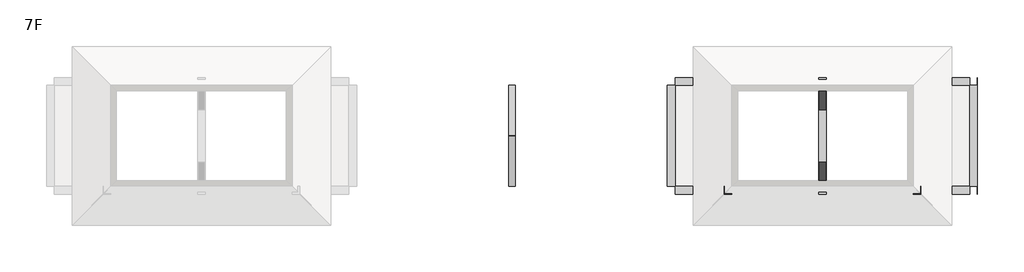
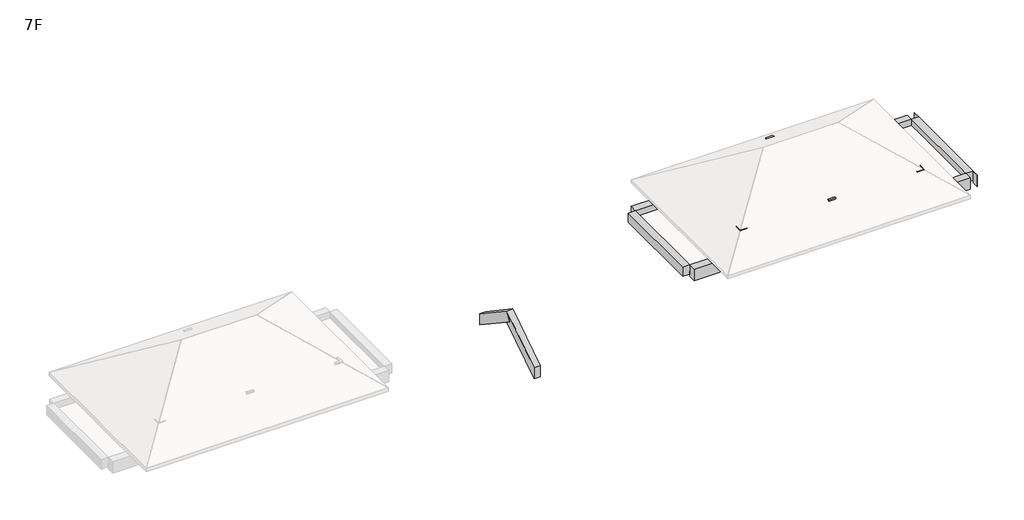
# One storey, part 2 of 2: 17 beams, 7 columns, 1 proxy.
"""IFC4 building model written with IfcOpenShell, lengths in millimetres."""

import ifcopenshell
import ifcopenshell.guid

model = None  # the IFC model being written
_history = None  # IfcOwnerHistory: only IFC2X3 demands one
_inside = {}  # id of a spatial element -> (the spatial element, [elements in it])
_under = {}  # id of a project, library or spatial element -> (it, [spatial elements below it])
_declared = {}  # id of a project -> (the project, [libraries it declares])
_typed = {}  # id of a type object -> (the type object, [elements of that type])
_made_of = {}  # id of a material, layer set ... -> (it, [elements and type objects made of it])


def new_model(schema):
    """Start an empty IFC model of exactly this schema.

    Asked for "IFC4X3", IfcOpenShell would pick the latest addendum, in which some entities
    have other attributes; the version numbers below select the first issue.
    IFC2X3 requires an IfcOwnerHistory on every rooted entity: one is made here for all.
    """
    global model, _history
    if schema == "IFC4X3":
        model = ifcopenshell.file(schema_version=(4, 3, 0, 0))
    else:
        model = ifcopenshell.file(schema=schema)
    _inside.clear()
    _under.clear()
    _declared.clear()
    _typed.clear()
    _made_of.clear()
    _history = None
    if model.schema == "IFC2X3":
        org = make("IfcOrganization", Name="unknown")
        user = make(
            "IfcPersonAndOrganization",
            ThePerson=make("IfcPerson", FamilyName="unknown"),
            TheOrganization=org,
        )
        app = make(
            "IfcApplication",
            ApplicationDeveloper=org,
            Version="unknown",
            ApplicationFullName="unknown",
            ApplicationIdentifier="unknown",
        )
        _history = make(
            "IfcOwnerHistory",
            OwningUser=user,
            OwningApplication=app,
            ChangeAction="ADDED",
            CreationDate=0,
        )
    return model


def make(cls, **values):
    """One entity of the class cls with the attributes given. An attribute that is None is left unset."""
    return model.create_entity(
        cls, **{name: value for name, value in values.items() if value is not None}
    )


def rooted(cls, **values):
    """An entity with a GlobalId (a new one), such as an element, a storey or a relation."""
    return make(cls, GlobalId=ifcopenshell.guid.new(), OwnerHistory=_history, **values)


def si_unit(unit_type, name, prefix=None):
    """IfcSIUnit, for example si_unit("LENGTHUNIT", "METRE", prefix="MILLI")."""
    return make("IfcSIUnit", UnitType=unit_type, Prefix=prefix, Name=name)


def assignment(units):
    """IfcUnitAssignment: the units of a project."""
    return None if units is None else make("IfcUnitAssignment", Units=units)


def point(xyz):
    """IfcCartesianPoint."""
    return None if xyz is None else make("IfcCartesianPoint", Coordinates=xyz)


def direction(xyz):
    """IfcDirection."""
    return None if xyz is None else make("IfcDirection", DirectionRatios=xyz)


def frame(location, z_axis=None, x_axis=None):
    """IfcAxis2Placement3D, a coordinate frame: its origin and axes. An axis left out is left unset."""
    return make(
        "IfcAxis2Placement3D",
        Location=point(location),
        Axis=direction(z_axis),
        RefDirection=direction(x_axis),
    )


def frame_2d(location, x_axis=None):
    """IfcAxis2Placement2D, a coordinate frame in the plane: its origin and x axis."""
    return make(
        "IfcAxis2Placement2D", Location=point(location), RefDirection=direction(x_axis)
    )


def origin():
    """The frame at (0, 0, 0) with its axes left unset."""
    return frame((0.0, 0.0, 0.0))


def origin_with_axes():
    """The frame at (0, 0, 0) with the z axis (0, 0, 1) and the x axis (1, 0, 0) written out."""
    return frame((0.0, 0.0, 0.0), z_axis=(0.0, 0.0, 1.0), x_axis=(1.0, 0.0, 0.0))


def place(relative_to, where):
    """IfcLocalPlacement: puts the frame where relative to a parent placement (None: the world)."""
    return make(
        "IfcLocalPlacement", PlacementRelTo=relative_to, RelativePlacement=where
    )


def context(
    kind, dimensions, precision=None, world=None, true_north=None, identifier=None
):
    """IfcGeometricRepresentationContext, for example the 3D "Model" context."""
    return make(
        "IfcGeometricRepresentationContext",
        ContextIdentifier=identifier,
        ContextType=kind,
        CoordinateSpaceDimension=dimensions,
        Precision=precision,
        WorldCoordinateSystem=world,
        TrueNorth=true_north,
    )


def project(units=None, contexts=None):
    """IfcProject with its units and contexts."""
    return rooted(
        "IfcProject",
        Name="project",
        RepresentationContexts=contexts,
        UnitsInContext=assignment(units),
    )


def spatial(cls, under=None, at=None, **own):
    """A site, building, storey or space (cls), placed at a placement, below another one or the project."""
    s = rooted(cls, ObjectPlacement=at, **own)
    if under is not None:
        _under.setdefault(under.id(), (under, []))[1].append(s)
    return s


def polyline(points):
    """IfcPolyline through the points."""
    return make("IfcPolyline", Points=[point(p) for p in points])


def circle_curve(where, radius):
    """IfcCircle in the frame where."""
    return make("IfcCircle", Position=where, Radius=radius)


def ellipse_curve(where, semi_axis1, semi_axis2):
    """IfcEllipse in the frame where."""
    return make(
        "IfcEllipse", Position=where, SemiAxis1=semi_axis1, SemiAxis2=semi_axis2
    )


def trimmed(basis, trim1, trim2, sense, master):
    """IfcTrimmedCurve: the piece of a basis curve between two trims."""
    return make(
        "IfcTrimmedCurve",
        BasisCurve=basis,
        Trim1=trim1,
        Trim2=trim2,
        SenseAgreement=sense,
        MasterRepresentation=master,
    )


def segment(curve, same_sense, transition):
    """IfcCompositeCurveSegment."""
    return make(
        "IfcCompositeCurveSegment",
        Transition=transition,
        SameSense=same_sense,
        ParentCurve=curve,
    )


def composite_curve(segments, self_intersect=None):
    """IfcCompositeCurve: segments joined end to end."""
    return make("IfcCompositeCurve", Segments=segments, SelfIntersect=self_intersect)


def outline(outer, holes=None, kind="AREA"):
    """IfcArbitraryClosedProfileDef: a profile drawn as a closed curve; with holes, ...WithVoids."""
    if holes is None:
        return make("IfcArbitraryClosedProfileDef", ProfileType=kind, OuterCurve=outer)
    return make(
        "IfcArbitraryProfileDefWithVoids",
        ProfileType=kind,
        OuterCurve=outer,
        InnerCurves=holes,
    )


def extrude(swept, where, along, depth):
    """IfcExtrudedAreaSolid: the profile swept, set in the frame where, extruded along a direction by depth."""
    return make(
        "IfcExtrudedAreaSolid",
        SweptArea=swept,
        Position=where,
        ExtrudedDirection=direction(along),
        Depth=depth,
    )


def faces_of(points, faces, orient=None, outer=None):
    """IfcFace entities. A face is a list of loops; a loop is a list of indices into points, from 0.

    orient and outer hold one flag for each loop. By default every Orientation is true, the
    first loop of a face is its IfcFaceOuterBound and the others are IfcFaceBound.
    """
    made = []
    for i, loops in enumerate(faces):
        bounds = []
        for j, loop in enumerate(loops):
            is_outer = j == 0 if outer is None else outer[i][j]
            bounds.append(
                make(
                    "IfcFaceOuterBound" if is_outer else "IfcFaceBound",
                    Bound=make("IfcPolyLoop", Polygon=[points[k] for k in loop]),
                    Orientation=True if orient is None else orient[i][j],
                )
            )
        made.append(make("IfcFace", Bounds=bounds))
    return made


def faceted_brep(points, faces, orient=None, outer=None, voids=None):
    """IfcFacetedBrep: a solid bounded by flat faces; with voids (closed shells), ...WithVoids."""
    shared = [point(p) for p in points]
    hull = make("IfcClosedShell", CfsFaces=faces_of(shared, faces, orient, outer))
    if voids is None:
        return make("IfcFacetedBrep", Outer=hull)
    return make(
        "IfcFacetedBrepWithVoids",
        Outer=hull,
        Voids=[
            make(cls, CfsFaces=faces_of(shared, fs, o, b)) for cls, fs, o, b in voids
        ],
    )


def shape(context_of_items, identifier, shape_type, items):
    """IfcShapeRepresentation: the items that make up one representation, for example the "Body"."""
    return make(
        "IfcShapeRepresentation",
        ContextOfItems=context_of_items,
        RepresentationIdentifier=identifier,
        RepresentationType=shape_type,
        Items=items,
    )


def source(mapping_origin, context_of_items, identifier, shape_type, items):
    """IfcRepresentationMap: a shape defined once, which mapped items show again and again."""
    return make(
        "IfcRepresentationMap",
        MappingOrigin=mapping_origin,
        MappedRepresentation=shape(context_of_items, identifier, shape_type, items),
    )


def transform(
    local_origin,
    x_axis=None,
    y_axis=None,
    z_axis=None,
    scale=None,
    scale2=None,
    scale3=None,
    uniform=True,
):
    """IfcCartesianTransformationOperator3D, or its non-uniform kind. x_axis, y_axis, z_axis: its Axis1, 2, 3."""
    if uniform:
        return make(
            "IfcCartesianTransformationOperator3D",
            Axis1=direction(x_axis),
            Axis2=direction(y_axis),
            LocalOrigin=point(local_origin),
            Scale=scale,
            Axis3=direction(z_axis),
        )
    return make(
        "IfcCartesianTransformationOperator3DnonUniform",
        Axis1=direction(x_axis),
        Axis2=direction(y_axis),
        LocalOrigin=point(local_origin),
        Scale=scale,
        Axis3=direction(z_axis),
        Scale2=scale2,
        Scale3=scale3,
    )


def mapped(mapping_source, mapping_target):
    """IfcMappedItem: shows the shape of a source again, moved by a transform."""
    return make(
        "IfcMappedItem", MappingSource=mapping_source, MappingTarget=mapping_target
    )


def made_of(thing, what):
    """Note that an element or type object is made of a material, layer set ...; save() writes the relation."""
    if what is not None:
        _made_of.setdefault(what.id(), (what, []))[1].append(thing)
    return thing


def element(
    cls,
    number,
    at=None,
    inside=None,
    cuts=None,
    type_object=None,
    material=None,
    context=None,
    identifier="Body",
    shape_type=None,
    held_by="IfcProductDefinitionShape",
    body=None,
    shapes=None,
    **own,
):
    """One element of the class cls, such as IfcWall. Its Tag is "e" and its number.

    at: its placement. inside: the storey or other place that contains it. cuts: it is an
    opening in that element (IfcRelVoidsElement). A single representation is given by context,
    identifier, shape_type and body (its items); several are given by shapes. held_by: the class
    of the entity that holds the representations. save() writes the other relations.
    """
    e = rooted(cls, Tag="e%d" % number, ObjectPlacement=at, **own)
    if body is not None:
        shapes = [shape(context, identifier, shape_type, body)]
    if shapes is not None:
        e.Representation = make(held_by, Representations=shapes)
    if inside is not None:
        _inside.setdefault(inside.id(), (inside, []))[1].append(e)
    if cuts is not None:
        rooted(
            "IfcRelVoidsElement", RelatingBuildingElement=cuts, RelatedOpeningElement=e
        )
    if type_object is not None:
        _typed.setdefault(type_object.id(), (type_object, []))[1].append(e)
    return made_of(e, material)


def aggregate(whole, parts):
    """IfcRelAggregates: a whole, such as a stair, and the parts it consists of."""
    return rooted("IfcRelAggregates", RelatingObject=whole, RelatedObjects=parts)


def save(model, path):
    """Write the relations noted so far, then the file.

    IfcRelAggregates (storeys below a building ...), IfcRelContainedInSpatialStructure (elements
    in a storey), IfcRelDefinesByType, IfcRelAssociatesMaterial and IfcRelDeclares: one each for
    every whole, place, type object, material and project.
    """
    for whole, parts in _under.values():
        aggregate(whole, parts)
    for where, things in _inside.values():
        rooted(
            "IfcRelContainedInSpatialStructure",
            RelatedElements=things,
            RelatingStructure=where,
        )
    for kind, things in _typed.values():
        rooted("IfcRelDefinesByType", RelatedObjects=things, RelatingType=kind)
    for what, things in _made_of.values():
        rooted("IfcRelAssociatesMaterial", RelatedObjects=things, RelatingMaterial=what)
    for by, libraries in _declared.values():
        rooted("IfcRelDeclares", RelatingContext=by, RelatedDefinitions=libraries)
    model.write(path)


def plane_surface(at):
    """IfcPlane: the flat surface through the origin of the frame at, square to its z axis."""
    return make("IfcPlane", Position=at)


def cylinder_surface(at, radius):
    """IfcCylindricalSurface: all points at the distance radius from the z axis of the frame at."""
    return make("IfcCylindricalSurface", Position=at, Radius=radius)


def revolved_surface(curve, axis_point, axis_direction):
    """IfcSurfaceOfRevolution: the curve turned about the line through axis_point along axis_direction."""
    return make(
        "IfcSurfaceOfRevolution",
        SweptCurve=make("IfcArbitraryOpenProfileDef", ProfileType="CURVE", Curve=curve),
        AxisPosition=make("IfcAxis1Placement", Location=point(axis_point), Axis=direction(axis_direction)),
    )


def advanced_brep(points, edges, surfaces, faces):
    """IfcAdvancedBrep: a solid bounded by faces that lie on surfaces and meet in shared edges.

    An edge is (start, end): straight between two places in points (the first is 0);
    or (start, end, curve); or (start, end, curve, False) where it runs against its curve.
    A face is (place in surfaces, loops), or (place, loops, False) where it looks against
    its surface's normal. A loop lists edges by number (the first is 1), with a minus sign
    where the edge is run from its end to its start. The first loop is the outer one.
    """
    corners = [point(p) for p in points]
    vertices = [make("IfcVertexPoint", VertexGeometry=c) for c in corners]
    made = []
    for start, end, *more in edges:
        made.append(
            make(
                "IfcEdgeCurve",
                EdgeStart=vertices[start],
                EdgeEnd=vertices[end],
                EdgeGeometry=more[0] if more else make("IfcPolyline", Points=[corners[start], corners[end]]),
                SameSense=more[1] if len(more) > 1 else True,
            )
        )
    hull = []
    for where, loops, *sense in faces:
        bounds = []
        for j, loop in enumerate(loops):
            ring = [make("IfcOrientedEdge", EdgeElement=made[abs(k) - 1], Orientation=k > 0) for k in loop]
            bounds.append(
                make(
                    "IfcFaceOuterBound" if j == 0 else "IfcFaceBound",
                    Bound=make("IfcEdgeLoop", EdgeList=ring),
                    Orientation=True,
                )
            )
        hull.append(make("IfcAdvancedFace", Bounds=bounds, FaceSurface=surfaces[where], SameSense=sense[0] if sense else True))
    return make("IfcAdvancedBrep", Outer=make("IfcClosedShell", CfsFaces=hull))


def m_support_metal_circular_m_support_metal_circular_a779fbb7(model_context):
    return source(origin(), model_context, "Body", "SolidModel", [
        advanced_brep(
        [(-6.0, 0.0, 0.0), (6.0, 0.0, 0.0), (-6.0, 0.0, -63.0), (6.0, 0.0, -63.0), (6.0, 12.0, -75.0), (-6.0, 12.0, -75.0), (-6.0, 63.0, -75.0), (6.0, 63.0, -75.0)],
        [
            (0, 1, circle_curve(origin_with_axes(), 6.0)),
            (1, 0, circle_curve(origin_with_axes(), 6.0)),
            (0, 2),
            (2, 3, circle_curve(frame((0.0, 0.0, -63.0), z_axis=(0.0, 0.0, 1.0), x_axis=(1.0, 0.0, 0.0)), 6.0)),
            (3, 1),
            (3, 2, circle_curve(frame((0.0, 0.0, -63.0), z_axis=(0.0, 0.0, 1.0), x_axis=(1.0, 0.0, 0.0)), 6.0)),
            (4, 3, circle_curve(frame((6.0, 12.0, -63.0), z_axis=(-1.0, 0.0, 0.0), x_axis=(0.0, -1.0, 0.0)), 12.0)),
            (2, 5, circle_curve(frame((-6.0, 12.0, -63.0), z_axis=(1.0, 0.0, 0.0), x_axis=(0.0, -1.0, 0.0)), 12.0)),
            (5, 4, circle_curve(frame((0.0, 12.0, -75.0), z_axis=(0.0, -1.0, 0.0), x_axis=(1.0, 0.0, 0.0)), 6.0)),
            (4, 5, circle_curve(frame((0.0, 12.0, -75.0), z_axis=(0.0, -1.0, 0.0), x_axis=(1.0, 0.0, 0.0)), 6.0)),
            (6, 7, circle_curve(frame((0.0, 63.0, -75.0), z_axis=(0.0, 1.0, 0.0), x_axis=(1.0, 0.0, 0.0)), 6.0)),
            (7, 6, circle_curve(frame((0.0, 63.0, -75.0), z_axis=(0.0, 1.0, 0.0), x_axis=(1.0, 0.0, 0.0)), 6.0)),
            (5, 6),
            (7, 4),
        ],
        [
            plane_surface(origin_with_axes()),
            cylinder_surface(origin_with_axes(), 6.0),
            revolved_surface(trimmed(ellipse_curve(frame((0.0, 0.0, -63.0), z_axis=(0.0, 0.0, 1.0), x_axis=(1.0, 0.0, 0.0)), 6.0, 6.0), [point((-6.0, 0.0, -63.0))], [point((6.0, 0.0, -63.0))], True, "CARTESIAN"), (0.0, 12.0, -63.0), (1.0, 0.0, 0.0)),
            revolved_surface(trimmed(ellipse_curve(frame((0.0, 0.0, -63.0), z_axis=(0.0, 0.0, 1.0), x_axis=(1.0, 0.0, 0.0)), 6.0, 6.0), [point((6.0, 0.0, -63.0))], [point((-6.0, 0.0, -63.0))], True, "CARTESIAN"), (0.0, 12.0, -63.0), (1.0, 0.0, 0.0)),
            plane_surface(frame((0.0, 63.0, -75.0), z_axis=(0.0, 1.0, 0.0), x_axis=(1.0, 0.0, 0.0))),
            cylinder_surface(frame((0.0, 12.0, -75.0), z_axis=(0.0, -1.0, 0.0), x_axis=(1.0, 0.0, 0.0)), 6.0),
        ],
        [
            (0, [[1, 2]]),
            (1, [[-1, 3, 4, 5]]),
            (1, [[-2, -5, 6, -3]]),
            (2, [[7, -4, 8, 9]]),
            (3, [[-8, -6, -7, 10]]),
            (4, [[11, 12]]),
            (5, [[-9, 13, -12, 14]]),
            (5, [[-10, -14, -11, -13]]),
        ],
    ),
        extrude(outline(composite_curve([segment(trimmed(circle_curve(frame_2d((-75.0, 0.0)), 25.0), [point((-75.0, -25.0))], [point((-75.0, 25.0))], False, "CARTESIAN"), True, "CONTINUOUS"), segment(trimmed(circle_curve(frame_2d((-75.0, 0.0)), 25.0), [point((-75.0, 25.0))], [point((-75.0, -25.0))], False, "CARTESIAN"), True, "CONTINUOUS")], self_intersect=False)), frame((0.0, 63.0, 0.0), z_axis=(0.0, 1.0, 0.0), x_axis=(0.0, 0.0, 1.0)), (0.0, 0.0, 1.0), 12.0),
    ])


model = new_model("IFC4")

# Units and contexts
model_context = context("Model", 3, world=origin())
ifc_project = project(units=[si_unit("LENGTHUNIT", "METRE", prefix="MILLI")], contexts=[model_context])

# Site, building, storey
site = spatial("IfcSite", under=ifc_project)
building = spatial("IfcBuilding", under=site)
storey = spatial("IfcBuildingStorey", under=building, Name="7F", Elevation=20530.0)

# Beams
placement = place(None, origin())
element("IfcBeam", 1, ObjectType="M_Concrete-Rectangular Beam : 250x400", at=placement, inside=storey, context=model_context, shape_type="Brep", body=[
    faceted_brep([(17975.0000046, 8450.0000002, 18285.6270793), (17725.0000046, 8450.0000002, 18285.6270793), (17725.0000046, 6499.7375861, 19585.8347272), (17975.0000046, 6499.7375861, 19585.8347272), (17725.0000046, 8450.0000002, 17804.8831884), (17725.0000046, 6499.7375861, 19105.0908362), (17725.0000046, 6277.8536437, 19253.0171854), (17975.0000046, 8450.0000002, 17804.8831884), (17975.0000046, 6499.7375861, 19105.0908362), (17975.0000046, 6277.8536437, 19253.0171854)], [[[0, 1, 2, 3]], [[4, 5, 6, 2, 1]], [[6, 5, 4, 7, 8, 9]], [[3, 9, 8, 7, 0]], [[1, 0, 7, 4]], [[3, 2, 6, 9]]]),
])
element("IfcBeam", 2, ObjectType="M_Concrete-Rectangular Beam : 250x400", at=placement, inside=storey, context=model_context, shape_type="SweptSolid", body=[
    extrude(outline(polyline([(33399.8746483, 8449.9999997), (33649.8746483, 8449.9999997), (33649.8746483, 4549.9999996), (33399.8746483, 4549.9999996), (33399.8746483, 8449.9999997)])), frame((0.0, 0.0, 20130.0), z_axis=(0.0, 0.0, 1.0), x_axis=(1.0, 0.0, 0.0)), (0.0, 0.0, 1.0), 400.0),
])
element("IfcBeam", 3, ObjectType="M_Concrete-Rectangular Beam : 250x400", at=placement, inside=storey, context=model_context, shape_type="SweptSolid", body=[
    extrude(outline(polyline([(26050.1253733, 8449.9999997), (26300.1253733, 8449.9999997), (26300.1253733, 4549.9999996), (26050.1253733, 4549.9999996), (26050.1253733, 8449.9999997)])), frame((0.0, 0.0, 20130.0), z_axis=(0.0, 0.0, 1.0), x_axis=(1.0, 0.0, 0.0)), (0.0, 0.0, 1.0), 400.0),
])
element("IfcBeam", 4, ObjectType="M_Concrete-Rectangular Beam : 250x400", at=placement, inside=storey, context=model_context, shape_type="SweptSolid", body=[
    extrude(outline(polyline([(4550.0000005, 18285.9769737), (6499.7375861, 19585.8347272), (6277.8536437, 19253.0171854), (6499.7375861, 19105.0908362), (4550.0000005, 17805.2330827), (4550.0000005, 18285.9769737)])), frame((17725.0000046, 0.0, 0.0), z_axis=(1.0, 0.0, 0.0), x_axis=(0.0, 1.0, 0.0)), (0.0, 0.0, 1.0), 250.0),
])
element("IfcBeam", 5, ObjectType="M_Concrete-Rectangular Beam : 250x400", at=placement, inside=storey, context=model_context, shape_type="Brep", body=[
    faceted_brep([(29725.0000715, 6499.7375861, 22885.8347272), (29975.0000715, 6499.7375861, 22885.8347272), (29975.0000715, 8449.9999997, 21585.6270796), (29725.0000715, 8449.9999997, 21585.6270796), (29725.0000715, 6277.8536437, 22553.0171854), (29725.0000715, 8449.9999997, 21104.8831887), (29725.0000715, 6499.7375861, 22405.0908362), (29975.0000715, 6277.8536437, 22553.0171854), (29975.0000715, 8449.9999997, 21104.8831887), (29975.0000715, 6499.7375861, 22405.0908362)], [[[0, 1, 2, 3]], [[4, 0, 3, 5, 6]], [[7, 4, 6, 5, 8, 9]], [[1, 7, 9, 8, 2]], [[1, 0, 4, 7]], [[3, 2, 8, 5]]]),
])
element("IfcBeam", 6, ObjectType="M_Concrete-Rectangular Beam : 250x400", at=placement, inside=storey, context=model_context, shape_type="SweptSolid", body=[
    extrude(outline(polyline([(6277.8536437, 22553.0171854), (6499.7375861, 22405.0908362), (4549.9999992, 21105.2330819), (4549.9999992, 21585.9769728), (6499.7375861, 22885.8347272), (6277.8536437, 22553.0171854)])), frame((29725.0000715, 0.0, 0.0), z_axis=(1.0, 0.0, 0.0), x_axis=(0.0, 1.0, 0.0)), (0.0, 0.0, 1.0), 250.0),
])
element("IfcBeam", 7, ObjectType="M_Concrete-Rectangular Beam : 250x400", at=placement, inside=storey, context=model_context, shape_type="Brep", body=[
    faceted_brep([(33629.982566, 4549.9999992, 21480.0), (33629.982566, 8724.9999993, 21480.0), (33625.119648, 8724.9999993, 21480.0), (33508.5592163, 8608.4366337, 21480.0), (33379.982566, 8608.4366337, 21480.0), (33379.982566, 8474.9999993, 21480.0), (33379.982566, 4549.9999992, 21480.0), (33379.982566, 4549.9999992, 21080.0), (33379.982566, 8655.7227157, 21448.4751524), (33379.982566, 8474.9999993, 21448.4751524), (33379.982566, 8449.9999997, 21448.4751524), (33379.982566, 8449.9999997, 21080.0), (33629.982566, 4549.9999992, 21080.0), (33629.982566, 8449.9999997, 21080.0), (33629.982566, 8449.9999997, 21448.4751524), (33629.982566, 8724.9999993, 21448.4751524), (33625.119648, 8724.9999993, 21448.4751524), (33555.8441081, 8655.7227157, 21448.4751524)], [[[0, 1, 2, 3, 4, 5, 6]], [[7, 6, 5, 4, 8, 9, 10, 11]], [[12, 7, 11, 13]], [[1, 0, 12, 13, 14, 15]], [[1, 15, 16, 2]], [[0, 6, 7, 12]], [[10, 14, 13, 11]], [[14, 10, 9, 8, 17, 16, 15]], [[3, 17, 8, 4]], [[17, 3, 2, 16]]]),
])
element("IfcBeam", 8, ObjectType="M_Concrete-Rectangular Beam : 250x400", at=placement, inside=storey, context=model_context, shape_type="SweptSolid", body=[
    extrude(outline(polyline([(21080.0, 26075.0175606), (21080.0, 26325.0175606), (21480.0, 26325.0175606), (21480.0, 26191.5713244), (21402.3014348, 26075.0175606), (21080.0, 26075.0175606)])), frame((0.0, 4549.9999992, 0.0), z_axis=(0.0, 1.0, 0.0), x_axis=(0.0, 0.0, 1.0)), (0.0, 0.0, 1.0), 3887.3000005),
])
element("IfcBeam", 9, ObjectType="M_Concrete-Rectangular Beam : 250x400", at=placement, inside=storey, context=model_context, shape_type="Brep", body=[
    faceted_brep([(29999.9855437, 8474.9999993, 21480.0), (33379.982566, 8474.9999993, 21480.0), (33379.982566, 8608.4366337, 21480.0), (29999.9855437, 8608.4366337, 21480.0), (33379.982566, 8474.9999993, 21448.4751524), (29999.9855437, 8474.9999993, 21080.0), (33349.8746414, 8474.9999993, 21080.0), (33349.8746414, 8474.9999993, 21448.4751524), (33349.8746414, 8724.9999993, 21080.0), (29999.9855437, 8724.9999993, 21080.0), (29999.9855437, 8724.9999993, 21402.2891349), (33349.8746414, 8724.9999993, 21402.2891349), (33379.982566, 8655.7227157, 21448.4751524), (33349.8746414, 8655.7227157, 21448.4751524)], [[[0, 1, 2, 3]], [[4, 1, 0, 5, 6, 7]], [[8, 6, 5, 9]], [[8, 9, 10, 11]], [[1, 4, 12, 2]], [[7, 6, 8, 11, 13]], [[4, 7, 13, 12]], [[5, 0, 3, 10, 9]], [[3, 2, 12, 13, 11, 10]]]),
    faceted_brep([(26075.0175606, 8474.9999993, 21448.4751524), (26075.0175606, 8474.9999993, 21480.0), (26075.0175606, 8724.7509238, 21480.0), (26075.0175606, 8724.7509238, 21448.4751524), (26350.1253663, 8474.9999993, 21080.0), (26350.1253663, 8474.9999993, 21448.4751524), (26350.1253663, 8655.7227157, 21448.4751524), (26350.1253663, 8724.9999993, 21402.2891349), (26350.1253663, 8724.9999993, 21080.0), (26144.0475062, 8655.7227157, 21448.4751524), (29699.9855437, 8474.9999993, 21480.0), (29699.9855437, 8474.9999993, 21080.0), (29699.9855437, 8724.9999993, 21080.0), (29699.9855437, 8724.9999993, 21402.2891349), (29699.9855437, 8608.4366337, 21480.0), (26191.3347784, 8608.4366337, 21480.0)], [[[0, 1, 2, 3]], [[4, 5, 6, 7, 8]], [[5, 0, 3, 9, 6]], [[10, 11, 12, 13, 14]], [[1, 10, 14, 15, 2]], [[1, 0, 5, 4, 11, 10]], [[4, 8, 12, 11]], [[12, 8, 7, 13]], [[15, 9, 3, 2]], [[9, 15, 14, 13, 7, 6]]]),
])
element("IfcBeam", 10, ObjectType="M_Concrete-Rectangular Beam : 250x400", at=placement, inside=storey, context=model_context, shape_type="SweptSolid", body=[
    extrude(outline(polyline([(4524.9999902, 21080.0), (4274.9999902, 21080.0), (4274.9999902, 21402.6390255), (4391.0385331, 21480.0), (4524.9999902, 21480.0), (4524.9999902, 21080.0)])), frame((29999.9855437, 0.0, 0.0), z_axis=(1.0, 0.0, 0.0), x_axis=(0.0, 1.0, 0.0)), (0.0, 0.0, 1.0), 3349.8890977),
    extrude(outline(polyline([(4524.9999902, 21480.0), (4524.9999902, 21080.0), (4274.9999902, 21080.0), (4274.9999902, 21402.6390255), (4391.0385331, 21480.0), (4524.9999902, 21480.0)])), frame((26350.0175606, 0.0, 0.0), z_axis=(1.0, 0.0, 0.0), x_axis=(0.0, 1.0, 0.0)), (0.0, 0.0, 1.0), 3349.9679831),
])
element("IfcBeam", 11, ObjectType="M_Concrete-Rectangular Beam : 300x400", at=placement, inside=storey, context=model_context, shape_type="Brep", body=[
    faceted_brep([(30000.0000031, 8449.9999997, 20530.0), (29999.533537, 8449.9999997, 20530.0), (29700.0000031, 8449.9999997, 20530.0), (29700.0000031, 4549.9999996, 20530.0), (29999.533537, 4549.9999996, 20530.0), (30000.0000031, 4549.9999996, 20530.0), (29700.0000031, 8449.9999997, 20130.0), (29700.0000031, 4549.9999996, 20130.0), (30000.0000031, 8449.9999997, 20130.0), (30000.0000031, 4549.9999996, 20130.0)], [[[0, 1, 2, 3, 4, 5]], [[2, 6, 7, 3]], [[6, 8, 9, 7]], [[8, 0, 5, 9]], [[2, 1, 0, 8, 6]], [[5, 4, 3, 7, 9]]]),
])
element("IfcBeam", 12, ObjectType="M_Concrete-Rectangular Beam : 300x400", at=placement, inside=storey, context=model_context, shape_type="Brep", body=[
    faceted_brep([(35835.035019, 8449.9999997, 20530.0), (35834.4843149, 8449.9999997, 20530.0), (35535.035019, 8449.9999997, 20530.0), (35535.035019, 4549.9999996, 20530.0), (35834.4843149, 4549.9999996, 20530.0), (35835.035019, 4549.9999996, 20530.0), (35535.035019, 8449.9999997, 20130.0), (35535.035019, 4549.9999996, 20130.0), (35835.035019, 8449.9999997, 20130.0), (35835.035019, 4549.9999996, 20130.0)], [[[0, 1, 2, 3, 4, 5]], [[2, 6, 7, 3]], [[6, 8, 9, 7]], [[8, 0, 5, 9]], [[2, 1, 0, 8, 6]], [[5, 4, 3, 7, 9]]]),
])
element("IfcBeam", 13, ObjectType="M_Concrete-Rectangular Beam : 300x400", at=placement, inside=storey, context=model_context, shape_type="Brep", body=[
    faceted_brep([(24149.9825174, 8449.9999997, 20530.0), (24149.516027, 8449.9999997, 20530.0), (23849.9825174, 8449.9999997, 20530.0), (23849.9825174, 4550.0000005, 20530.0), (24149.516027, 4549.9999996, 20530.0), (24149.9825174, 4549.9999996, 20530.0), (23849.9825174, 8449.9999997, 20130.0), (23849.9825174, 4550.0000005, 20130.0), (24149.9825174, 8449.9999997, 20130.0), (24149.9825174, 4549.9999996, 20130.0)], [[[0, 1, 2, 3, 4, 5]], [[2, 6, 7, 3]], [[6, 8, 9, 7]], [[8, 0, 5, 9]], [[2, 1, 0, 8, 6]], [[3, 7, 9, 5, 4]]]),
])
element("IfcBeam", 14, ObjectType="M_Concrete-Rectangular Beam : 300x500", at=placement, inside=storey, context=model_context, shape_type="Brep", body=[
    faceted_brep([(30000.0000031, 8449.9999997, 20530.0), (30000.0000031, 8749.9999997, 20530.0), (29999.533537, 8749.9999997, 20530.0), (29999.533537, 8449.9999997, 20530.0), (30000.0000031, 8449.9999997, 20030.0), (30000.0000031, 8449.9999997, 20130.0), (29999.533537, 8449.9999997, 20030.0), (30000.0000031, 8749.9999997, 20030.0), (29999.533537, 8749.9999997, 20030.0)], [[[0, 1, 2, 3]], [[4, 5, 0, 3, 6]], [[7, 4, 6, 8]], [[1, 7, 8, 2]], [[1, 0, 5, 4, 7]], [[3, 2, 8, 6]]]),
    faceted_brep([(24149.516027, 8449.9999997, 20530.0), (24149.516027, 8749.9999997, 20530.0), (24149.516027, 8749.9999997, 20030.0), (24149.516027, 8449.9999997, 20030.0), (29699.533537, 8749.9999997, 20530.0), (29699.533537, 8449.9999997, 20530.0), (29699.533537, 8449.9999997, 20030.0), (29699.533537, 8749.9999997, 20030.0), (24149.9825174, 8449.9999997, 20530.0), (26050.1253733, 8449.9999997, 20530.0), (26300.1253733, 8449.9999997, 20530.0), (26350.1253663, 8449.9999997, 20530.0), (26350.1253663, 8749.9999997, 20530.0), (26050.1253663, 8749.9999997, 20530.0)], [[[0, 1, 2, 3]], [[4, 5, 6, 7]], [[1, 0, 8, 9, 10, 11, 5, 4, 12, 13]], [[0, 3, 6, 5, 11, 10, 9, 8]], [[3, 2, 7, 6]], [[2, 1, 13, 12, 4, 7]]]),
])
element("IfcBeam", 15, ObjectType="M_Concrete-Rectangular Beam : 300x500", at=placement, inside=storey, context=model_context, shape_type="Brep", body=[
    faceted_brep([(30000.0000031, 4249.9999996, 20530.0), (30000.0000031, 4549.9999996, 20530.0), (29999.533537, 4549.9999996, 20530.0), (29999.533537, 4249.9999996, 20530.0), (30000.0000031, 4249.9999996, 20030.0), (29999.533537, 4249.9999996, 20030.0), (30000.0000031, 4549.9999996, 20030.0), (29999.533537, 4549.9999996, 20030.0), (30000.0000031, 4549.9999996, 20130.0)], [[[0, 1, 2, 3]], [[4, 0, 3, 5]], [[6, 4, 5, 7]], [[1, 8, 6, 7, 2]], [[1, 0, 4, 6, 8]], [[3, 2, 7, 5]]]),
    faceted_brep([(24149.516027, 4249.9999996, 20530.0), (24149.516027, 4549.9999996, 20530.0), (24149.516027, 4549.9999996, 20030.0), (24149.516027, 4249.9999996, 20030.0), (29699.533537, 4549.9999996, 20530.0), (29699.533537, 4249.9999996, 20530.0), (29699.533537, 4249.9999996, 20030.0), (29699.533537, 4549.9999996, 20030.0), (26300.1253733, 4549.9999996, 20530.0), (26050.1253733, 4549.9999996, 20530.0), (24149.9825174, 4549.9999996, 20530.0)], [[[0, 1, 2, 3]], [[4, 5, 6, 7]], [[1, 0, 5, 4, 8, 9, 10]], [[0, 3, 6, 5]], [[3, 2, 7, 6]], [[2, 1, 10, 9, 8, 4, 7]]]),
])
element("IfcBeam", 16, ObjectType="M_Concrete-Rectangular Beam : 300x500", at=placement, inside=storey, context=model_context, shape_type="Brep", body=[
    faceted_brep([(35835.035019, 8449.9999997, 20530.0), (35835.035019, 8749.9999997, 20530.0), (35834.4843149, 8749.9999997, 20530.0), (35834.4843149, 8449.9999997, 20530.0), (35835.035019, 8449.9999997, 20030.0), (35835.035019, 8449.9999997, 20130.0), (35834.4843149, 8449.9999997, 20030.0), (35835.035019, 8749.9999997, 20030.0), (35834.4843149, 8749.9999997, 20030.0)], [[[0, 1, 2, 3]], [[4, 5, 0, 3, 6]], [[7, 4, 6, 8]], [[1, 7, 8, 2]], [[1, 0, 5, 4, 7]], [[3, 2, 8, 6]]]),
    faceted_brep([(35534.4843149, 8749.9999997, 20530.0), (35534.4843149, 8449.9999997, 20530.0), (35534.4843149, 8449.9999997, 20030.0), (35534.4843149, 8749.9999997, 20030.0), (30000.0000031, 8449.9999997, 20530.0), (30000.0000031, 8749.9999997, 20530.0), (30000.0000031, 8749.9999997, 20030.0), (30000.0000031, 8449.9999997, 20030.0), (33349.8746414, 8449.9999997, 20530.0), (33399.8746483, 8449.9999997, 20530.0), (33649.8746483, 8449.9999997, 20530.0), (33649.8746414, 8749.9999997, 20530.0), (33349.8746414, 8749.9999997, 20530.0)], [[[0, 1, 2, 3]], [[4, 5, 6, 7]], [[5, 4, 8, 9, 10, 1, 0, 11, 12]], [[4, 7, 2, 1, 10, 9, 8]], [[7, 6, 3, 2]], [[6, 5, 12, 11, 0, 3]]]),
])
element("IfcBeam", 17, ObjectType="M_Concrete-Rectangular Beam : 300x500", at=placement, inside=storey, context=model_context, shape_type="Brep", body=[
    faceted_brep([(35835.035019, 4249.9999996, 20530.0), (35835.035019, 4549.9999996, 20530.0), (35834.4843149, 4549.9999996, 20530.0), (35834.4843149, 4249.9999996, 20530.0), (35835.035019, 4249.9999996, 20030.0), (35834.4843149, 4249.9999996, 20030.0), (35835.035019, 4549.9999996, 20030.0), (35834.4843149, 4549.9999996, 20030.0), (35835.035019, 4549.9999996, 20130.0)], [[[0, 1, 2, 3]], [[4, 0, 3, 5]], [[6, 4, 5, 7]], [[1, 8, 6, 7, 2]], [[1, 0, 4, 6, 8]], [[3, 2, 7, 5]]]),
    faceted_brep([(30000.0000031, 4249.9999996, 20530.0), (30000.0000031, 4549.9999996, 20530.0), (30000.0000031, 4549.9999996, 20030.0), (30000.0000031, 4249.9999996, 20030.0), (35534.4843149, 4549.9999996, 20530.0), (35534.4843149, 4249.9999996, 20530.0), (35534.4843149, 4249.9999996, 20030.0), (35534.4843149, 4549.9999996, 20030.0), (33649.8746483, 4549.9999996, 20530.0), (33399.8746483, 4549.9999996, 20530.0)], [[[0, 1, 2, 3]], [[4, 5, 6, 7]], [[5, 4, 8, 9, 1, 0]], [[6, 5, 0, 3]], [[7, 6, 3, 2]], [[4, 7, 2, 1, 9, 8]]]),
])

# Proxy
m_support_metal_circular_m_support_metal_circular_shape = m_support_metal_circular_m_support_metal_circular_a779fbb7(model_context)
element("IfcBuildingElementProxy", 18, Name="M_Support - Metal - Circular : M_Support - Metal - Circular", ObjectType="M_Support - Metal - Circular : M_Support - Metal - Circular", at=placement, inside=storey, context=model_context, shape_type="MappedRepresentation", body=[
    mapped(m_support_metal_circular_m_support_metal_circular_shape, transform((4604.999959, 3949.9999996, 20530.0), x_axis=(1.0, 0.0, 0.0), y_axis=(0.0, 1.0, 0.0), z_axis=(0.0, 0.0, 1.0))),
])

# Columns
element("IfcColumn", 19, ObjectType="M_Concrete-Rectangular-Column : 300x300", at=placement, inside=storey, context=model_context, shape_type="SweptSolid", body=[
    extrude(outline(polyline([(9649.8746382, 8749.9999997), (9649.8746382, 8449.9999997), (9349.8746382, 8449.9999997), (9349.8746382, 8749.9999997), (9649.8746382, 8749.9999997)])), frame((0.0, 0.0, 20530.0), z_axis=(0.0, 0.0, 1.0), x_axis=(1.0, 0.0, 0.0)), (0.0, 0.0, 1.0), 918.4751524),
])
element("IfcColumn", 20, ObjectType="M_Concrete-Rectangular-Column : 300x300", at=placement, inside=storey, context=model_context, shape_type="Brep", body=[
    faceted_brep([(29999.9855437, 4549.9999992, 20530.0), (29999.9855437, 4249.9999992, 20530.0), (29699.9855437, 4249.9999992, 20530.0), (29699.9855437, 4549.9999992, 20530.0), (29699.9855437, 4549.9999992, 21585.9769764), (29999.9855437, 4549.9999992, 21585.9769764), (29999.9855437, 4249.9999992, 21385.9719455), (29999.9855437, 4274.9999902, 21402.6390255), (29999.9855437, 4391.0385331, 21480.0), (29699.9855437, 4391.0385331, 21480.0), (29699.9855437, 4274.9999902, 21402.6390255), (29699.9855437, 4249.9999992, 21385.9719455)], [[[0, 1, 2, 3]], [[0, 3, 4, 5]], [[6, 7, 8, 5, 4, 9, 10, 11]], [[1, 0, 5, 8, 7, 6]], [[2, 1, 6, 11]], [[3, 2, 11, 10, 9, 4]]]),
    faceted_brep([(29999.9855437, 4249.9999992, 21585.9769764), (29999.9855437, 4249.9999992, 21530.1951128), (29999.9855437, 4333.6706899, 21585.9769764), (29699.9855437, 4249.9999992, 21585.9769764), (29699.9855437, 4249.9999992, 21530.1951128), (29699.9855437, 4333.6706899, 21585.9769764)], [[[0, 1, 2]], [[0, 3, 4, 1]], [[4, 3, 5]], [[3, 0, 2, 5]], [[2, 1, 4, 5]]]),
])
element("IfcColumn", 21, ObjectType="M_Concrete-Rectangular-Column : 300x300", at=placement, inside=storey, context=model_context, shape_type="Brep", body=[
    faceted_brep([(29999.9855437, 8749.9999997, 20530.0), (29999.9855437, 8449.9999997, 20530.0), (29999.533537, 8449.9999997, 20530.0), (29699.9855437, 8449.9999997, 20530.0), (29699.9855437, 8749.9999997, 20530.0), (29999.533537, 8749.9999997, 20530.0), (29999.9855437, 8449.9999997, 21585.6270796), (29699.9855437, 8449.9999997, 21585.6270796), (29999.9855437, 8608.4366337, 21480.0), (29999.9855437, 8724.9999993, 21402.2891349), (29999.9855437, 8749.9999997, 21385.6220487), (29699.9855437, 8749.9999997, 21385.6220487), (29699.9855437, 8724.9999993, 21402.2891349), (29699.9855437, 8608.4366337, 21480.0)], [[[0, 1, 2, 3, 4, 5]], [[3, 2, 1, 6, 7]], [[6, 8, 9, 10, 11, 12, 13, 7]], [[1, 0, 10, 9, 8, 6]], [[4, 3, 7, 13, 12, 11]], [[0, 5, 4, 11, 10]]]),
    faceted_brep([(29999.9855437, 8749.9999997, 21529.845216), (29999.9855437, 8749.9999997, 21585.6270796), (29999.9855437, 8666.329309, 21585.6270796), (29699.9855437, 8749.9999997, 21585.6270796), (29699.9855437, 8749.9999997, 21529.845216), (29699.9855437, 8666.329309, 21585.6270796)], [[[0, 1, 2]], [[3, 4, 5]], [[3, 1, 0, 4]], [[1, 3, 5, 2]], [[0, 2, 5, 4]]]),
])
element("IfcColumn", 22, ObjectType="M_Concrete-Rectangular-Column : 300x300", at=placement, inside=storey, context=model_context, shape_type="Brep", body=[
    faceted_brep([(33649.8746414, 4549.9999992, 20530.0), (33649.8746414, 4249.9999992, 20530.0), (33349.8746414, 4249.9999992, 20530.0), (33349.8746414, 4549.9999992, 20530.0), (33649.8746414, 4549.9999992, 21544.0553738), (33649.8746414, 4249.9999992, 21544.0553738), (33649.8746414, 4249.9999992, 21529.9272796), (33649.8746414, 4549.9999992, 21529.9272796), (33649.8746414, 4249.9999992, 21385.7074809), (33649.5942023, 4249.9999992, 21385.8944308), (33649.5942023, 4249.9999992, 21530.1142294), (33349.8746414, 4249.9999992, 21544.0553738), (33349.8746414, 4549.9999992, 21544.0553738), (33628.6814244, 4549.9999992, 21544.0553738), (33628.6814244, 4270.9133035, 21544.0553738), (33412.3407455, 4487.2594281, 21544.0553738), (33412.3407455, 4549.9999992, 21544.0553738), (33649.8746414, 4549.9999992, 21385.7074809)], [[[0, 1, 2, 3]], [[4, 5, 6, 7]], [[2, 1, 8, 9, 10, 6, 5, 11]], [[3, 2, 11, 12]], [[4, 7, 13]], [[5, 4, 13, 14, 15, 16, 12, 11]], [[15, 9, 8, 17, 16]], [[10, 14, 13, 7, 6]], [[9, 15, 14, 10]], [[1, 0, 17, 8]], [[0, 3, 12, 16, 17]]]),
])
element("IfcColumn", 23, ObjectType="M_Concrete-Rectangular-Column : 300x300", at=placement, inside=storey, context=model_context, shape_type="Brep", body=[
    faceted_brep([(33649.8746414, 8749.9999997, 20530.0), (33649.8746414, 8449.9999997, 20530.0), (33349.8746414, 8449.9999997, 20530.0), (33349.8746414, 8749.9999997, 20530.0), (33649.8746414, 8749.9999997, 21385.6220487), (33649.8746414, 8749.7556157, 21385.7849755), (33649.8746414, 8749.7556157, 21448.4751524), (33649.8746414, 8449.9999997, 21448.4751524), (33349.8746414, 8449.9999997, 21448.4751524), (33349.8746414, 8655.7227157, 21448.4751524), (33349.8746414, 8749.9999997, 21385.6220487), (33555.8441081, 8655.7227157, 21448.4751524)], [[[0, 1, 2, 3]], [[1, 0, 4, 5, 6, 7]], [[2, 1, 7, 8]], [[3, 2, 8, 9, 10]], [[0, 3, 10, 4]], [[8, 7, 6, 11, 9]], [[11, 5, 4, 10, 9]], [[5, 11, 6]]]),
])
element("IfcColumn", 24, ObjectType="M_Concrete-Rectangular-Column : 300x300", at=placement, inside=storey, context=model_context, shape_type="Brep", body=[
    faceted_brep([(26350.1253663, 4549.9999992, 20530.0), (26350.1253663, 4249.9999992, 20530.0), (26050.1253663, 4249.9999992, 20530.0), (26050.1253663, 4549.9999992, 20530.0), (26350.1253663, 4549.9999992, 21544.0553738), (26350.1253663, 4249.9999992, 21544.0553738), (26050.1253663, 4249.9999992, 21544.0553738), (26050.1253663, 4249.9999992, 21529.9272796), (26050.4058054, 4249.9999992, 21530.1142294), (26050.4058054, 4249.9999992, 21385.8944308), (26050.1253663, 4249.9999992, 21385.7074809), (26050.1253663, 4549.9999992, 21544.0553738), (26050.1253663, 4549.9999992, 21529.9272796), (26071.3185833, 4549.9999992, 21544.0553738), (26287.6592622, 4549.9999992, 21544.0553738), (26287.6592622, 4487.2594281, 21544.0553738), (26071.3185833, 4270.9133035, 21544.0553738), (26050.1253663, 4549.9999992, 21385.7074809)], [[[0, 1, 2, 3]], [[1, 0, 4, 5]], [[2, 1, 5, 6, 7, 8, 9, 10]], [[6, 11, 12, 7]], [[12, 11, 13]], [[5, 4, 14, 15, 16, 13, 11, 6]], [[9, 15, 14, 17, 10]], [[16, 8, 7, 12, 13]], [[15, 9, 8, 16]], [[3, 2, 10, 17]], [[0, 3, 17, 14, 4]]]),
])
element("IfcColumn", 25, ObjectType="M_Concrete-Rectangular-Column : 300x300", at=placement, inside=storey, context=model_context, shape_type="Brep", body=[
    faceted_brep([(26350.1253663, 8749.9999997, 20530.0), (26350.1253663, 8449.9999997, 20530.0), (26050.1253663, 8449.9999997, 20530.0), (26050.1253663, 8749.9999997, 20530.0), (26350.1253663, 8749.9999997, 21385.6220487), (26350.1253663, 8655.7227157, 21448.4751524), (26350.1253663, 8449.9999997, 21448.4751524), (26050.1253663, 8449.9999997, 21448.4751524), (26050.1253663, 8749.6424915, 21448.4751524), (26050.1253663, 8749.6424915, 21385.8603935), (26050.1253663, 8749.9999997, 21385.6220487), (26144.0475062, 8655.7227157, 21448.4751524)], [[[0, 1, 2, 3]], [[1, 0, 4, 5, 6]], [[2, 1, 6, 7]], [[3, 2, 7, 8, 9, 10]], [[0, 3, 10, 4]], [[7, 6, 5, 11, 8]], [[9, 11, 5, 4, 10]], [[11, 9, 8]]]),
])

save(model, "model.ifc")

# Revit data of these elements
# Type "M_Concrete-Rectangular Beam : 250x400"
#   Length [instance default] = 1524 mm
#   b = 250 mm
#   h = 400 mm
#   Structural Material [instance default] = Concrete, Cast-in-Place gray
#   Assembly Code = ""
# Type "M_Concrete-Rectangular Beam : 300x400"
#   Length [instance default] = 1524 mm
#   b = 300 mm
#   h = 400 mm
#   Structural Material [instance default] = Concrete, Cast-in-Place gray
#   Assembly Code = ""
# Type "M_Concrete-Rectangular Beam : 300x500"
#   Length [instance default] = 1524 mm
#   b = 300 mm
#   h = 500 mm
#   Structural Material [instance default] = Concrete, Cast-in-Place gray
#   Assembly Code = ""
# Type "M_Support - Metal - Circular : M_Support - Metal - Circular"
#   T1 = 12 mm
#   Radius 2 = 6 mm
#   Radius 1 = 25 mm
#   built-in parameter 1152166 = 0.246063 (stored number, unit not read)
#   built-in parameter 1152165 [instance default] = 0.246063 (stored number, unit not read)
#   Bend Radius = 12 mm
#   Support Material = Aluminum
# Type "M_Concrete-Rectangular-Column : 300x300"
#   b = 300 mm
#   h = 300 mm
#   Structural Material [instance default] = Concrete, Cast-in-Place gray
# Elements 1, 4, 5, 6 (IfcBeam, "M_Concrete-Rectangular Beam : 250x400")
#   Comments = ""
#   COF_CON__WorkItemNumber = "SH3-A-03F"
#   COF_GEN__Name = "DM3"
#   Structural Material = Concrete, Cast-in-Place gray
#   Phase Created = New Construction
#   Materials on its faces: "Concrete, Cast-in-Place gray"
# Elements 2, 3 (IfcBeam, "M_Concrete-Rectangular Beam : 250x400")
#   Comments = ""
#   COF_CON__WorkItemNumber = "SH3-A-03F"
#   COF_GEN__Name = "DT2"
#   Structural Material = Concrete, Cast-in-Place gray
#   Phase Created = New Construction
#   Materials on its faces: "Concrete, Cast-in-Place gray"
# Elements 7, 8 (IfcBeam, "M_Concrete-Rectangular Beam : 250x400")
#   Comments = ""
#   COF_CON__WorkItemNumber = "SH3-A-03F"
#   COF_GEN__Name = "DM2"
#   Structural Material = Concrete, Cast-in-Place gray
#   Phase Created = New Construction
#   Materials on its faces: "Concrete, Cast-in-Place gray"
# Elements 9, 10 (IfcBeam, "M_Concrete-Rectangular Beam : 250x400")
#   Comments = ""
#   COF_CON__WorkItemNumber = "SH3-A-03F"
#   COF_GEN__Name = "DM1"
#   Structural Material = Concrete, Cast-in-Place gray
#   Phase Created = New Construction
#   Materials on its faces: "Concrete, Cast-in-Place gray"
# Elements 11, 12, 13 (IfcBeam, "M_Concrete-Rectangular Beam : 300x400")
#   Comments = ""
#   COF_CON__WorkItemNumber = "SH3-A-03F"
#   COF_GEN__Name = "DT1"
#   Structural Material = Concrete, Cast-in-Place gray
#   Phase Created = New Construction
#   Materials on its faces: "Concrete, Cast-in-Place gray"
# Elements 14, 15, 16, 17 (IfcBeam, "M_Concrete-Rectangular Beam : 300x500")
#   Comments = ""
#   COF_CON__WorkItemNumber = "SH3-A-03F"
#   COF_GEN__Name = "D2A"
#   Structural Material = Concrete, Cast-in-Place gray
#   Phase Created = New Construction
#   Materials on its faces: "Concrete, Cast-in-Place gray"
# Element 18 (IfcBuildingElementProxy, "M_Support - Metal - Circular : M_Support - Metal - Circular")
#   built-in parameter 1152165 = 0.246063 (stored number, unit not read)
#   Materials on its faces: "Aluminum"
# Elements 19, 22, 23, 24, 25 (IfcColumn, "M_Concrete-Rectangular-Column : 300x300")
#   Comments = ""
#   COF_CON__WorkItemNumber = "SH3-A-TF"
#   COF_GEN__Name = "TR5"
#   Structural Material = Concrete, Cast-in-Place gray
#   Phase Created = New Construction
#   Materials on its faces: "Concrete, Cast-in-Place gray"
# Elements 20, 21 (IfcColumn, "M_Concrete-Rectangular-Column : 300x300")
#   Comments = ""
#   COF_CON__WorkItemNumber = "SH3-A-TF"
#   COF_GEN__Name = "TR4"
#   Structural Material = Concrete, Cast-in-Place gray
#   Phase Created = New Construction
#   Materials on its faces: "Concrete, Cast-in-Place gray"
# Materials
#   "Concrete, Cast-in-Place gray": class "Concrete", colour RGB 207 208 204, transparency 0, Description = "Cast-in-place concrete", Cost = 0
#   "Aluminum": class "Metal", colour RGB 247 247 247, transparency 0, Description = "Aluminum 6061", Cost = 0
